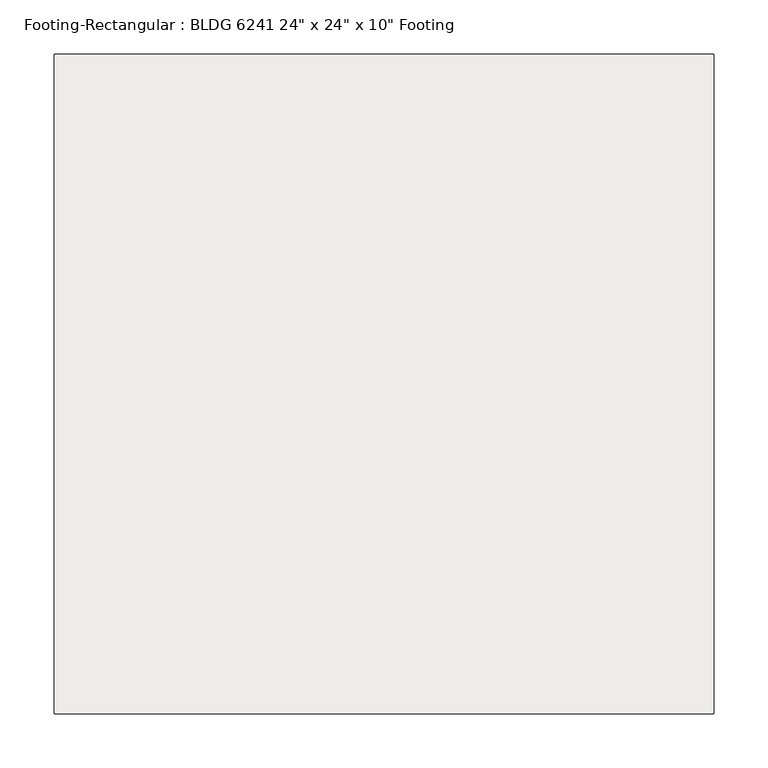
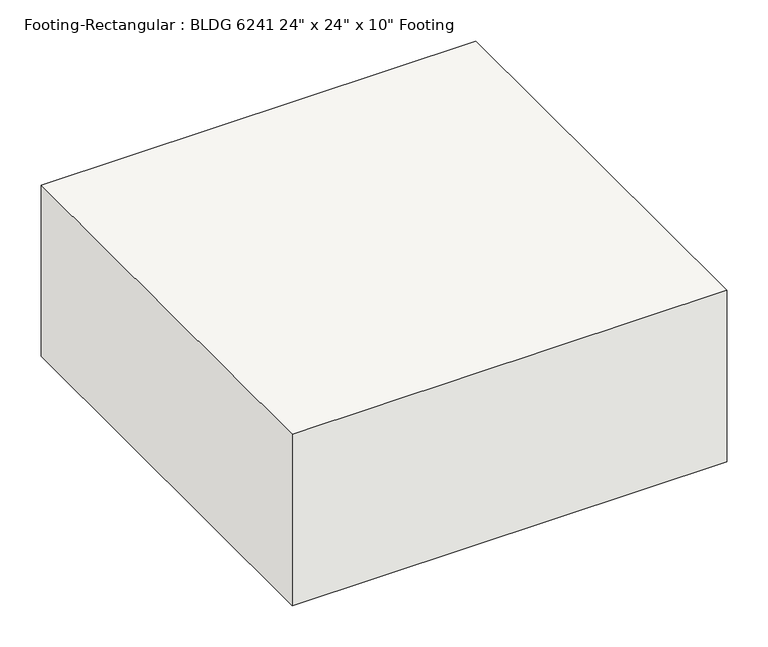
"""IFC4 building model written with IfcOpenShell, lengths in millimetres: slab geometry."""

from ifc_helpers import new_model, si_unit, frame, origin, place, context, project, spatial, polyline, outline, extrude, source, transform, mapped, element, save


def slab_7656c398(model_context):
    return source(origin(), model_context, "Body", "SweptSolid", [
        extrude(outline(polyline([(304.8, 304.8), (304.8, -304.8), (-304.8, -304.8), (-304.8, 304.8), (304.8, 304.8)])), frame((0.0, 0.0, -254.0), z_axis=(0.0, 0.0, 1.0), x_axis=(1.0, 0.0, 0.0)), (0.0, 0.0, 1.0), 254.0),
    ])


if __name__ == "__main__":
    model = new_model("IFC4")
    model_context = context("Model", 3, world=origin())
    ifc_project = project(units=[si_unit("LENGTHUNIT", "METRE", prefix="MILLI")], contexts=[model_context])
    site = spatial("IfcSite", under=ifc_project)
    building = spatial("IfcBuilding", under=site)
    placement = place(None, origin())
    slab_shape = slab_7656c398(model_context)
    element("IfcSlab", 1, ObjectType="Footing-Rectangular : BLDG 6241 24\" x 24\" x 10\" Footing", at=placement, inside=building, context=model_context, shape_type="MappedRepresentation", body=[
        mapped(slab_shape, transform((0.0, 0.0, 0.0), x_axis=(1.0, 0.0, 0.0), y_axis=(0.0, 1.0, 0.0), z_axis=(0.0, 0.0, 1.0))),
    ])
    save(model, "model.ifc")

# Revit data of these elements
# Type "Footing-Rectangular : BLDG 6241 24\" x 24\" x 10\" Footing"
#   Assembly Code = "A1010100"
#   Width = 2' - 0"
#   Length = 2' - 0"
#   Foundation Thickness = 0' - 10"
#   Structural Material [instance default] = Concrete, Cast-in-Place gray
# Element 1 (IfcSlab, "Footing-Rectangular : BLDG 6241 24\" x 24\" x 10\" Footing")
#   Structural Material = BLDG 6241 Concrete(3500 psi)
#   Materials on its faces: "BLDG 6241 Concrete(3500 psi)"
# Materials
#   "Concrete, Cast-in-Place gray": class "Concrete", colour RGB 192 192 192, transparency 0, Description = "Cast-in-place concrete", Cost = 0
#   "BLDG 6241 Concrete(3500 psi)": class "Concrete", colour RGB 127 127 127, transparency 0, Description = "Portland Cement Concrete", Cost = 0
